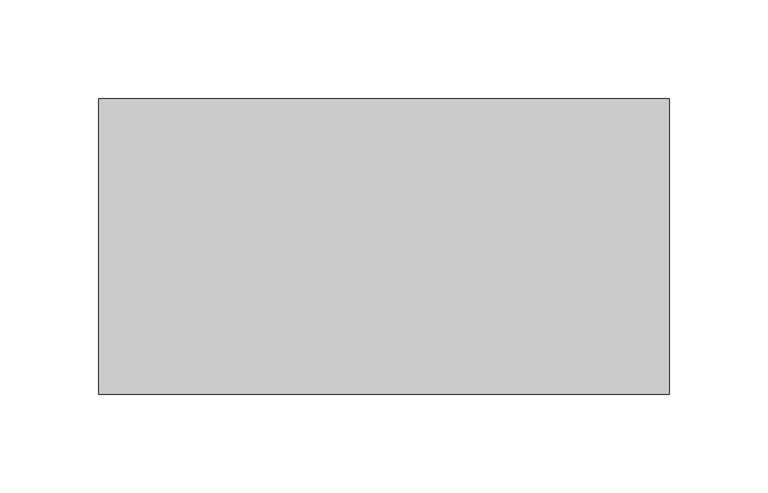
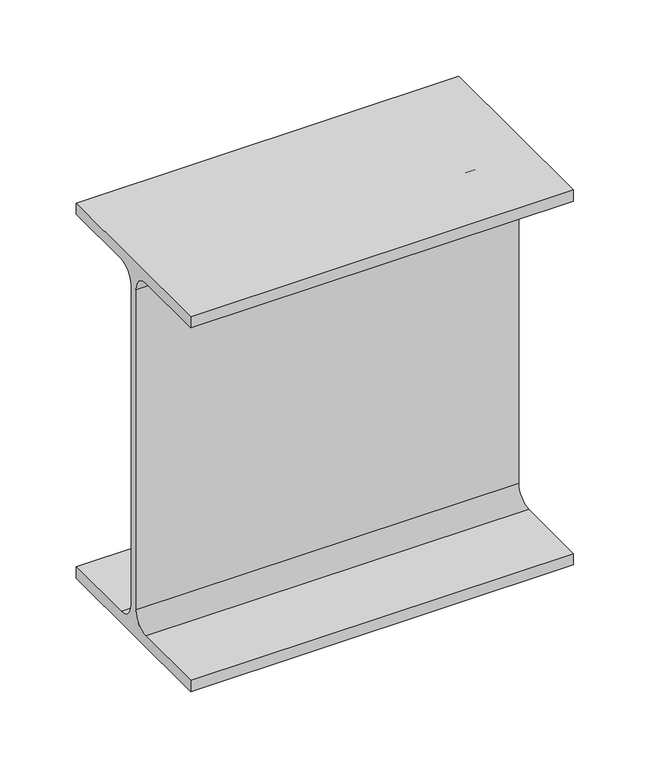
"""IFC4 building model written with IfcOpenShell, lengths in millimetres: beam geometry, 0912_Steel Framing_H-KSD3502 : H_SB_ASB_H-300x150x6.5x9."""

from ifc_helpers import new_model, si_unit, point, frame, frame_2d, origin, place, context, project, spatial, polyline, circle_curve, trimmed, segment, composite_curve, outline, extrude, source, transform, mapped, element, save


def beam_e857d536(model_context):
    return source(origin(), model_context, "Body", "SweptSolid", [
        extrude(outline(composite_curve([segment(polyline([(75.0, -141.0), (75.0, -150.0), (-75.0, -150.0), (-75.0, -141.0), (-16.25, -141.0)]), True, "CONTINUOUS"), segment(trimmed(circle_curve(frame_2d((-16.25, -128.0)), 13.0), [point((-16.25, -141.0))], [point((-3.25, -128.0))], True, "CARTESIAN"), True, "CONTINUOUS"), segment(polyline([(-3.25, -128.0), (-3.25, 128.0)]), True, "CONTINUOUS"), segment(trimmed(circle_curve(frame_2d((-16.25, 128.0)), 13.0), [point((-3.25, 128.0))], [point((-16.25, 141.0))], True, "CARTESIAN"), True, "CONTINUOUS"), segment(polyline([(-16.25, 141.0), (-75.0, 141.0), (-75.0, 150.0), (75.0, 150.0), (75.0, 141.0), (16.25, 141.0)]), True, "CONTINUOUS"), segment(trimmed(circle_curve(frame_2d((16.25, 128.0)), 13.0), [point((16.25, 141.0))], [point((3.25, 128.0))], True, "CARTESIAN"), True, "CONTINUOUS"), segment(polyline([(3.25, 128.0), (3.25, -128.0)]), True, "CONTINUOUS"), segment(trimmed(circle_curve(frame_2d((16.25, -128.0)), 13.0), [point((3.25, -128.0))], [point((16.25, -141.0))], True, "CARTESIAN"), True, "CONTINUOUS"), segment(polyline([(16.25, -141.0), (75.0, -141.0)]), True, "CONTINUOUS")], self_intersect=False)), frame((-7.3, 0.0, 0.0), z_axis=(1.0, 0.0, 0.0), x_axis=(0.0, 1.0, 0.0)), (0.0, 0.0, 1.0), 289.6),
    ])


if __name__ == "__main__":
    model = new_model("IFC4")
    model_context = context("Model", 3, world=origin())
    ifc_project = project(units=[si_unit("LENGTHUNIT", "METRE", prefix="MILLI")], contexts=[model_context])
    site = spatial("IfcSite", under=ifc_project)
    building = spatial("IfcBuilding", under=site)
    placement = place(None, origin())
    beam_shape = beam_e857d536(model_context)
    element("IfcBeam", 1, ObjectType="0912_Steel Framing_H-KSD3502 : H_SB_ASB_H-300x150x6.5x9", at=placement, inside=building, context=model_context, shape_type="MappedRepresentation", body=[
        mapped(beam_shape, transform((0.0, 0.0, 0.0), x_axis=(1.0, 0.0, 0.0), y_axis=(0.0, 1.0, 0.0), z_axis=(0.0, 0.0, 1.0))),
    ])
    save(model, "model.ifc")

# Revit data of these elements
# Type "0912_Steel Framing_H-KSD3502 : H_SB_ASB_H-300x150x6.5x9"
#   H_WM Code_1 = "S01AA002-00001 | Main Steel Structure Fabrication Work | Shelter/Building | Medium Steel - Standard (90KG/M>Weight≥30KG/M) | Material: (   )"
#   H_WM Code_2 = "S03AA028-00001 | Main Steel Structure Erection Work | Shelter/Building | Medium Steel (90KG/M>Weight≥30KG/M) | Material: (   )"
#   H_WM Code_3 = "S01AA010-00001 | Main Steel Structure Fabrication Work | Shelter/Building | Steel Painting/Coating | for Non-Fireproofed Steel Surface, Surface Preparation, Primer, Second & Final Coat | Material: (   )"
#   H_Q'ty Cal Type Tag = "SB-Q2"
#   Width = 15.0 cm
#   Web Thickness = 0.65 cm
#   Web Fillet = 1.3 cm
#   Warping Constant = 107000.0 cm⁶
#   W = 0
#   Torsional Moment of Inertia = 9.9539 cm⁴
#   Section Area = 46.78 cm²
#   Plastic Modulus weak axis = 105.0 cm³
#   Plastic Modulus strong axis = 542.0 cm³
#   Perimeter = 1.17 m²/m
#   Nominal Weight = 36.70 kgf/m
#   Moment of Inertia weak axis = 508.00 cm⁴
#   Moment of Inertia strong axis = 7210.00 cm⁴
#   Height = 30.0 cm
#   Flange Thickness = 0.9 cm
#   Elastic Modulus weak axis = 67.7 cm³
#   Elastic Modulus strong axis = 481.0 cm³
#   Centroid Vertical = 15.0 cm
#   Centroid Horizontal = 7.5 cm
#   Ix = 72100000
#   Length [instance default] = 1.5240 m
#   Zx = 542000
#   b = 0.1500 m
#   h = 0.3000 m
#   r = 0.0130 m
#   s = 0.0065 m
#   t = 0.0090 m
#   A = 0.004678 m²
#   Structural Material [instance default] = Steel, 45-345
#   Assembly Code = ""
# Element 1 (IfcBeam, "0912_Steel Framing_H-KSD3502 : H_SB_ASB_H-300x150x6.5x9")
#   Structural Material = none
# Materials
#   "Steel, 45-345": class "Metal", colour RGB 189 187 185, transparency 0, Description = "Steel 345 MPa", Cost = 0
